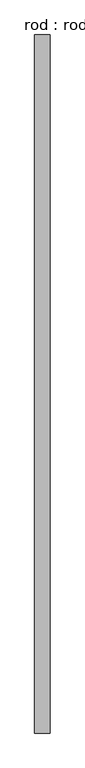
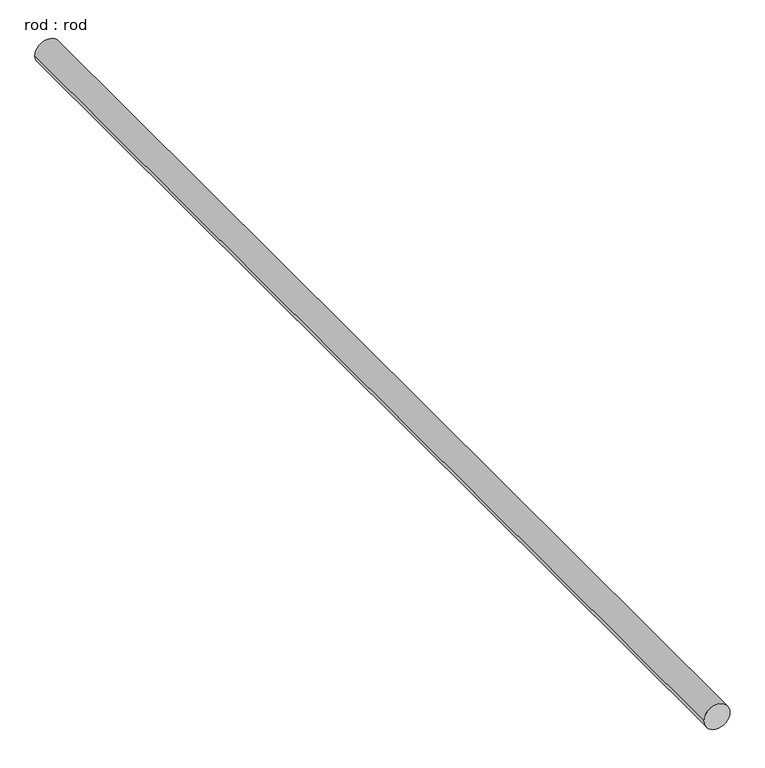
"""IFC4 building model written with IfcOpenShell, lengths in millimetres: proxy geometry, rod : rod."""

from ifc_helpers import new_model, si_unit, point, frame, frame_2d, origin, place, context, project, spatial, circle_curve, trimmed, segment, composite_curve, outline, extrude, source, transform, mapped, element, save


def rod_rod_b96c4223(model_context):
    return source(origin(), model_context, "Body", "SweptSolid", [
        extrude(outline(composite_curve([segment(trimmed(circle_curve(frame_2d((0.0108462, 0.0)), 200.0), [point((0.0108462, 200.0))], [point((0.0108462, -200.0))], False, "CARTESIAN"), True, "CONTINUOUS"), segment(trimmed(circle_curve(frame_2d((0.0108462, 0.0)), 200.0), [point((0.0108462, -200.0))], [point((0.0108462, 200.0))], False, "CARTESIAN"), True, "CONTINUOUS")], self_intersect=False)), frame((0.0, -4867.0928132, 0.0), z_axis=(0.0, 1.0, 0.0), x_axis=(0.0, 0.0, 1.0)), (0.0, 0.0, 1.0), 17919.6428571),
    ])


if __name__ == "__main__":
    model = new_model("IFC4")
    model_context = context("Model", 3, world=origin())
    ifc_project = project(units=[si_unit("LENGTHUNIT", "METRE", prefix="MILLI")], contexts=[model_context])
    site = spatial("IfcSite", under=ifc_project)
    building = spatial("IfcBuilding", under=site)
    placement = place(None, origin())
    rod_rod_shape = rod_rod_b96c4223(model_context)
    element("IfcBuildingElementProxy", 1, Name="rod : rod", ObjectType="rod : rod", at=placement, inside=building, context=model_context, shape_type="MappedRepresentation", body=[
        mapped(rod_rod_shape, transform((0.0, 0.0, 0.0), x_axis=(1.0, 0.0, 0.0), y_axis=(0.0, 1.0, 0.0), z_axis=(0.0, 0.0, 1.0))),
    ])
    save(model, "model.ifc")

# Revit data of these elements
# Type "rod : rod"
#   Default Elevation = 0
